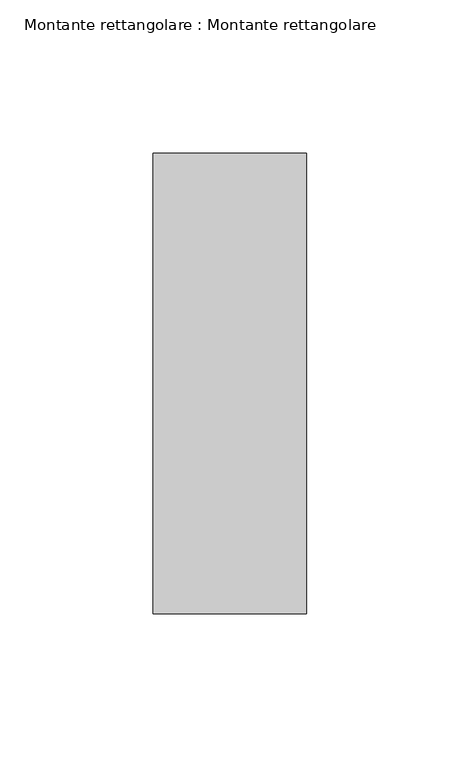
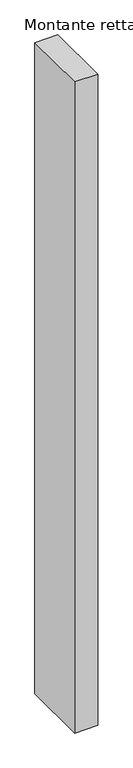
"""IFC4 building model written with IfcOpenShell, lengths in millimetres: member geometry, Montante rettangolare : Montante rettangolare."""

from ifc_helpers import new_model, si_unit, frame, origin, place, context, project, spatial, polyline, outline, extrude, source, transform, mapped, element, save


def montante_rettangolare_montante_rettangolare_461a195c(model_context):
    return source(origin(), model_context, "Body", "SweptSolid", [
        extrude(outline(polyline([(0.0, 75.0), (0.0, -75.0), (-50.0, -75.0), (-50.0, 75.0), (0.0, 75.0)])), frame((0.0, 0.0, -1500.0), z_axis=(0.0, 0.0, 1.0), x_axis=(1.0, 0.0, 0.0)), (0.0, 0.0, 1.0), 1500.0),
    ])


if __name__ == "__main__":
    model = new_model("IFC4")
    model_context = context("Model", 3, world=origin())
    ifc_project = project(units=[si_unit("LENGTHUNIT", "METRE", prefix="MILLI")], contexts=[model_context])
    site = spatial("IfcSite", under=ifc_project)
    building = spatial("IfcBuilding", under=site)
    placement = place(None, origin())
    montante_rettangolare_montante_rettangolare_shape = montante_rettangolare_montante_rettangolare_461a195c(model_context)
    element("IfcMember", 1, ObjectType="Montante rettangolare : Montante rettangolare", at=placement, inside=building, context=model_context, shape_type="MappedRepresentation", body=[
        mapped(montante_rettangolare_montante_rettangolare_shape, transform((0.0, 0.0, 0.0), x_axis=(1.0, 0.0, 0.0), y_axis=(0.0, 1.0, 0.0), z_axis=(0.0, 0.0, 1.0))),
    ])
    save(model, "model.ifc")

# Revit data of these elements
# Type "Montante rettangolare : Montante rettangolare"
#   built-in parameter 1007304 = 0.492126 (stored number, unit not read)
#   built-in parameter 1007301 = 0.082021 (stored number, unit not read)
#   built-in parameter 1007300 = 0.082021 (stored number, unit not read)
# Element 1 (IfcMember, "Montante rettangolare : Montante rettangolare")
#   Materials on its faces: "Acciaio"
# Materials
#   "Acciaio": class "Metallo", colour RGB 247 247 247, transparency 0, Description = "Acciaio, finitura zigrinata", Cost = 0
